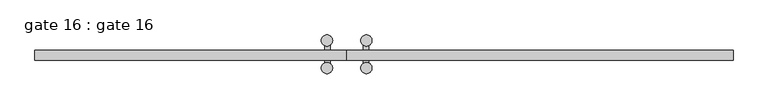
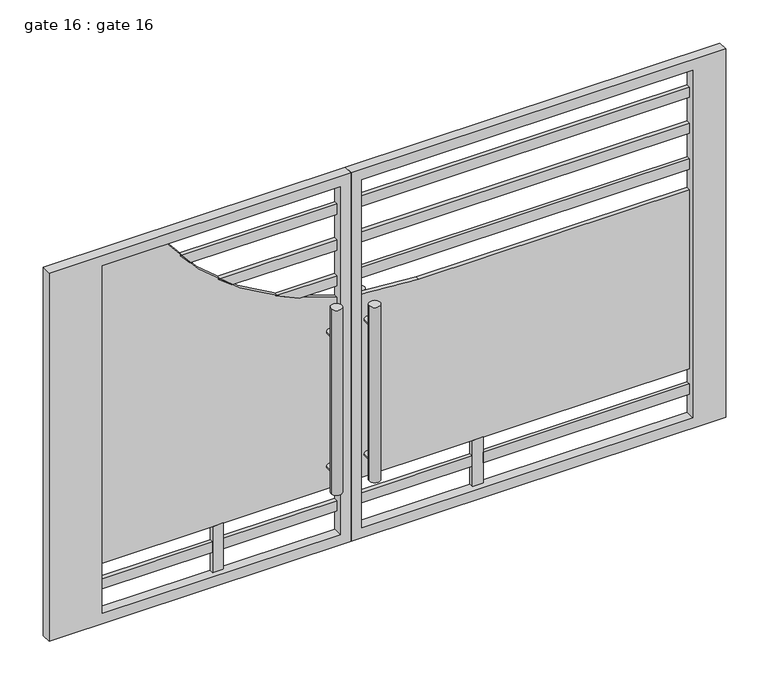
"""IFC4 building model written with IfcOpenShell, lengths in millimetres: proxy geometry, gate 16 : gate 16."""

from ifc_helpers import new_model, si_unit, point, frame, frame_2d, origin, place, context, project, spatial, polyline, circle_curve, trimmed, segment, composite_curve, outline, extrude, source, transform, mapped, element, save


def gate_16_gate_16_8623d773(model_context):
    return source(origin(), model_context, "Body", "SweptSolid", [
        extrude(outline(composite_curve([segment(trimmed(circle_curve(frame_2d((389.4541496, -88.119132)), 12.7), [point((389.4541496, -75.419132))], [point((389.4541496, -100.819132))], False, "CARTESIAN"), True, "CONTINUOUS"), segment(trimmed(circle_curve(frame_2d((389.4541496, -88.119132)), 12.7), [point((389.4541496, -100.819132))], [point((389.4541496, -75.419132))], False, "CARTESIAN"), True, "CONTINUOUS")], self_intersect=False)), frame((0.0, -57.15, 0.0), z_axis=(0.0, 1.0, 0.0), x_axis=(0.0, 0.0, 1.0)), (0.0, 0.0, 1.0), 76.7981605),
        extrude(outline(composite_curve([segment(trimmed(circle_curve(frame_2d((1058.3458504, -88.119132)), 12.7), [point((1058.3458504, -75.419132))], [point((1058.3458504, -100.819132))], False, "CARTESIAN"), True, "CONTINUOUS"), segment(trimmed(circle_curve(frame_2d((1058.3458504, -88.119132)), 12.7), [point((1058.3458504, -100.819132))], [point((1058.3458504, -75.419132))], False, "CARTESIAN"), True, "CONTINUOUS")], self_intersect=False)), frame((0.0, -57.15, 0.0), z_axis=(0.0, 1.0, 0.0), x_axis=(0.0, 0.0, 1.0)), (0.0, 0.0, 1.0), 76.6172039),
        extrude(outline(composite_curve([segment(trimmed(circle_curve(frame_2d((389.4541496, 88.119132)), 12.7), [point((389.4541496, 75.419132))], [point((389.4541496, 100.819132))], False, "CARTESIAN"), True, "CONTINUOUS"), segment(trimmed(circle_curve(frame_2d((389.4541496, 88.119132)), 12.7), [point((389.4541496, 100.819132))], [point((389.4541496, 75.419132))], False, "CARTESIAN"), True, "CONTINUOUS")], self_intersect=False)), frame((0.0, -57.15, 0.0), z_axis=(0.0, 1.0, 0.0), x_axis=(0.0, 0.0, 1.0)), (0.0, 0.0, 1.0), 76.7981605),
        extrude(outline(composite_curve([segment(trimmed(circle_curve(frame_2d((1058.3458504, 88.119132)), 12.7), [point((1058.3458504, 75.419132))], [point((1058.3458504, 100.819132))], False, "CARTESIAN"), True, "CONTINUOUS"), segment(trimmed(circle_curve(frame_2d((1058.3458504, 88.119132)), 12.7), [point((1058.3458504, 100.819132))], [point((1058.3458504, 75.419132))], False, "CARTESIAN"), True, "CONTINUOUS")], self_intersect=False)), frame((0.0, -57.15, 0.0), z_axis=(0.0, 1.0, 0.0), x_axis=(0.0, 0.0, 1.0)), (0.0, 0.0, 1.0), 76.6172039),
        extrude(outline(composite_curve([segment(trimmed(circle_curve(frame_2d((89.7949058, -81.8785099)), 25.4), [point((64.3949058, -81.8785099))], [point((115.1949058, -81.8785099))], False, "CARTESIAN"), True, "CONTINUOUS"), segment(trimmed(circle_curve(frame_2d((89.7949058, -81.8785099)), 25.4), [point((115.1949058, -81.8785099))], [point((64.3949058, -81.8785099))], False, "CARTESIAN"), True, "CONTINUOUS")], self_intersect=False)), frame((0.0, 0.0, 298.8472671), z_axis=(0.0, 0.0, 1.0), x_axis=(1.0, 0.0, 0.0)), (0.0, 0.0, 1.0), 869.5527329),
        extrude(outline(composite_curve([segment(trimmed(circle_curve(frame_2d((-89.7949058, -81.8785099)), 25.4), [point((-64.3949058, -81.8785099))], [point((-115.1949058, -81.8785099))], False, "CARTESIAN"), True, "CONTINUOUS"), segment(trimmed(circle_curve(frame_2d((-89.7949058, -81.8785099)), 25.4), [point((-115.1949058, -81.8785099))], [point((-64.3949058, -81.8785099))], False, "CARTESIAN"), True, "CONTINUOUS")], self_intersect=False)), frame((0.0, 0.0, 298.8472671), z_axis=(0.0, 0.0, 1.0), x_axis=(1.0, 0.0, 0.0)), (0.0, 0.0, 1.0), 917.3073645),
        extrude(outline(composite_curve([segment(trimmed(circle_curve(frame_2d((89.7949058, 43.7785099)), 25.4), [point((64.3949058, 43.7785099))], [point((115.1949058, 43.7785099))], False, "CARTESIAN"), True, "CONTINUOUS"), segment(trimmed(circle_curve(frame_2d((89.7949058, 43.7785099)), 25.4), [point((115.1949058, 43.7785099))], [point((64.3949058, 43.7785099))], False, "CARTESIAN"), True, "CONTINUOUS")], self_intersect=False)), frame((0.0, 0.0, 279.4), z_axis=(0.0, 0.0, 1.0), x_axis=(1.0, 0.0, 0.0)), (0.0, 0.0, 1.0), 889.0),
        extrude(outline(composite_curve([segment(trimmed(circle_curve(frame_2d((-89.7949058, 43.7785099)), 25.4), [point((-64.3949058, 43.7785099))], [point((-115.1949058, 43.7785099))], False, "CARTESIAN"), True, "CONTINUOUS"), segment(trimmed(circle_curve(frame_2d((-89.7949058, 43.7785099)), 25.4), [point((-115.1949058, 43.7785099))], [point((-64.3949058, 43.7785099))], False, "CARTESIAN"), True, "CONTINUOUS")], self_intersect=False)), frame((0.0, 0.0, 279.4), z_axis=(0.0, 0.0, 1.0), x_axis=(1.0, 0.0, 0.0)), (0.0, 0.0, 1.0), 889.0),
        extrude(outline(polyline([(-584.2, -19.05), (-635.0, -19.05), (-635.0, 0.0), (-584.2, 0.0), (-584.2, -19.05)])), frame((0.0, 0.0, 50.8), z_axis=(0.0, 0.0, 1.0), x_axis=(1.0, 0.0, 0.0)), (0.0, 0.0, 1.0), 228.6),
        extrude(outline(polyline([(635.0, -19.05), (584.2, -19.05), (584.2, 0.0), (635.0, 0.0), (635.0, -19.05)])), frame((0.0, 0.0, 50.8), z_axis=(0.0, 0.0, 1.0), x_axis=(1.0, 0.0, 0.0)), (0.0, 0.0, 1.0), 228.6),
        extrude(outline(polyline([(-635.0, -19.05), (-1168.4, -19.05), (-1168.4, 0.0), (-635.0, 0.0), (-635.0, -19.05)])), frame((0.0, 0.0, 152.4), z_axis=(0.0, 0.0, 1.0), x_axis=(1.0, 0.0, 0.0)), (0.0, 0.0, 1.0), 50.8),
        extrude(outline(polyline([(-50.8, -19.05), (-584.2, -19.05), (-584.2, 0.0), (-50.8, 0.0), (-50.8, -19.05)])), frame((0.0, 0.0, 152.4), z_axis=(0.0, 0.0, 1.0), x_axis=(1.0, 0.0, 0.0)), (0.0, 0.0, 1.0), 50.8),
        extrude(outline(polyline([(1604.0815715, -19.05), (635.0, -19.05), (635.0, 0.0), (1604.0815715, 0.0), (1604.0815715, -19.05)])), frame((0.0, 0.0, 152.4), z_axis=(0.0, 0.0, 1.0), x_axis=(1.0, 0.0, 0.0)), (0.0, 0.0, 1.0), 50.8),
        extrude(outline(polyline([(584.2, -19.05), (50.8, -19.05), (50.8, 0.0), (584.2, 0.0), (584.2, -19.05)])), frame((0.0, 0.0, 152.4), z_axis=(0.0, 0.0, 1.0), x_axis=(1.0, 0.0, 0.0)), (0.0, 0.0, 1.0), 50.8),
        extrude(outline(composite_curve([segment(polyline([(1676.4, -50.8), (1676.4, -786.3350015)]), True, "CONTINUOUS"), segment(trimmed(circle_curve(frame_2d((2582.6324877, 299.8877691)), 1414.6155764), [point((1676.4, -786.3350015))], [point((1625.6, -741.8540639))], False, "CARTESIAN"), True, "CONTINUOUS"), segment(polyline([(1625.6, -741.8540639), (1625.6, -50.8), (1676.4, -50.8)]), True, "CONTINUOUS")], self_intersect=False)), frame((0.0, -19.05, 0.0), z_axis=(0.0, 1.0, 0.0), x_axis=(0.0, 0.0, 1.0)), (0.0, 0.0, 1.0), 19.05),
        extrude(outline(polyline([(1604.0815715, -19.05), (50.8, -19.05), (50.8, 0.0), (1604.0815715, 0.0), (1604.0815715, -19.05)])), frame((0.0, 0.0, 1625.6), z_axis=(0.0, 0.0, 1.0), x_axis=(1.0, 0.0, 0.0)), (0.0, 0.0, 1.0), 50.8),
        extrude(outline(composite_curve([segment(polyline([(1498.6, -50.8), (1498.6, -608.963591)]), True, "CONTINUOUS"), segment(trimmed(circle_curve(frame_2d((2582.6324877, 299.8877691)), 1414.6155764), [point((1498.6, -608.963591))], [point((1447.8, -544.6786605))], False, "CARTESIAN"), True, "CONTINUOUS"), segment(polyline([(1447.8, -544.6786605), (1447.8, -50.8), (1498.6, -50.8)]), True, "CONTINUOUS")], self_intersect=False)), frame((0.0, -19.05, 0.0), z_axis=(0.0, 1.0, 0.0), x_axis=(0.0, 0.0, 1.0)), (0.0, 0.0, 1.0), 19.05),
        extrude(outline(polyline([(1604.0815715, -19.05), (50.8, -19.05), (50.8, 0.0), (1604.0815715, 0.0), (1604.0815715, -19.05)])), frame((0.0, 0.0, 1447.8), z_axis=(0.0, 0.0, 1.0), x_axis=(1.0, 0.0, 0.0)), (0.0, 0.0, 1.0), 50.8),
        extrude(outline(composite_curve([segment(polyline([(1320.8, -50.8), (1320.8, -339.5776342)]), True, "CONTINUOUS"), segment(trimmed(circle_curve(frame_2d((2582.6324877, 299.8877691)), 1414.6155764), [point((1320.8, -339.5776342))], [point((1270.0, -227.4955652))], False, "CARTESIAN"), True, "CONTINUOUS"), segment(polyline([(1270.0, -227.4955652), (1270.0, -50.8), (1320.8, -50.8)]), True, "CONTINUOUS")], self_intersect=False)), frame((0.0, -19.05, 0.0), z_axis=(0.0, 1.0, 0.0), x_axis=(0.0, 0.0, 1.0)), (0.0, 0.0, 1.0), 19.05),
        extrude(outline(polyline([(1604.0815715, -19.05), (50.8, -19.05), (50.8, 0.0), (1604.0815715, 0.0), (1604.0815715, -19.05)])), frame((0.0, 0.0, 1270.0), z_axis=(0.0, 0.0, 1.0), x_axis=(1.0, 0.0, 0.0)), (0.0, 0.0, 1.0), 50.8),
        extrude(outline(composite_curve([segment(polyline([(1778.0, -1168.4), (279.4, -1168.4), (279.4, -50.8), (1212.1744192, -50.8)]), True, "CONTINUOUS"), segment(trimmed(circle_curve(frame_2d((2582.6324877, 299.8877691)), 1414.6155764), [point((1212.1744192, -50.8))], [point((1778.0, -863.6))], True, "CARTESIAN"), True, "CONTINUOUS"), segment(polyline([(1778.0, -863.6), (1778.0, -1168.4)]), True, "CONTINUOUS")], self_intersect=False)), frame((0.0, -19.05, 0.0), z_axis=(0.0, 1.0, 0.0), x_axis=(0.0, 0.0, 1.0)), (0.0, 0.0, 1.0), 19.05),
        extrude(outline(composite_curve([segment(polyline([(279.4, 1604.0815715), (1168.4, 1604.0815715), (1168.4, 332.8073642)]), True, "CONTINUOUS"), segment(trimmed(circle_curve(frame_2d((2582.6324877, 299.8877691)), 1414.6155764), [point((1168.4, 332.8073642))], [point((1190.1194672, 50.8))], True, "CARTESIAN"), True, "CONTINUOUS"), segment(polyline([(1190.1194672, 50.8), (279.4, 50.8), (279.4, 1604.0815715)]), True, "CONTINUOUS")], self_intersect=False)), frame((0.0, -19.05, 0.0), z_axis=(0.0, 1.0, 0.0), x_axis=(0.0, 0.0, 1.0)), (0.0, 0.0, 1.0), 19.05),
        extrude(outline(polyline([(0.0, 1758.2918226), (1828.8, 1758.2918226), (1828.8, 0.0), (0.0, 0.0), (0.0, 1758.2918226)]), holes=[polyline([(50.8, 1604.0815715), (50.8, 50.8), (1778.0, 50.8), (1778.0, 1604.0815715), (50.8, 1604.0815715)])]), frame((0.0, -46.0617726, 0.0), z_axis=(0.0, 1.0, 0.0), x_axis=(0.0, 0.0, 1.0)), (0.0, 0.0, 1.0), 46.0617726),
        extrude(outline(polyline([(0.0, -1418.5646457), (0.0, 0.0), (1828.8, 0.0), (1828.8, -1418.5646457), (0.0, -1418.5646457)]), holes=[polyline([(50.8, -1168.4), (1778.0, -1168.4), (1778.0, -50.8), (50.8, -50.8), (50.8, -1168.4)])]), frame((0.0, -46.0617726, 0.0), z_axis=(0.0, 1.0, 0.0), x_axis=(0.0, 0.0, 1.0)), (0.0, 0.0, 1.0), 46.0617726),
    ])


if __name__ == "__main__":
    model = new_model("IFC4")
    model_context = context("Model", 3, world=origin())
    ifc_project = project(units=[si_unit("LENGTHUNIT", "METRE", prefix="MILLI")], contexts=[model_context])
    site = spatial("IfcSite", under=ifc_project)
    building = spatial("IfcBuilding", under=site)
    placement = place(None, origin())
    gate_16_gate_16_shape = gate_16_gate_16_8623d773(model_context)
    element("IfcBuildingElementProxy", 1, Name="gate 16 : gate 16", ObjectType="gate 16 : gate 16", at=placement, inside=building, context=model_context, shape_type="MappedRepresentation", body=[
        mapped(gate_16_gate_16_shape, transform((0.0, 0.0, 0.0), x_axis=(1.0, 0.0, 0.0), y_axis=(0.0, 1.0, 0.0), z_axis=(0.0, 0.0, 1.0))),
    ])
    save(model, "model.ifc")

# Revit data of these elements
# Type "gate 16 : gate 16"
#   sheet = none
#   pipe = METAL TEXTURE
#   handal = METAL TEXTURE
#   faram = none
#   SHEET-1 = STRIP
#   Default Elevation = 0
# Element 1 (IfcBuildingElementProxy, "gate 16 : gate 16")
#   Materials on its faces: "METAL TEXTURE", "STRIP"
# Materials
#   "METAL TEXTURE": class "Generic", colour RGB 120 120 120, transparency 0, Cost = 0
#   "STRIP": class "Generic", colour RGB 120 120 120, transparency 0, Cost = 0
